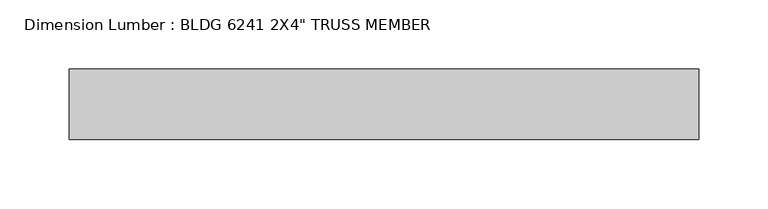
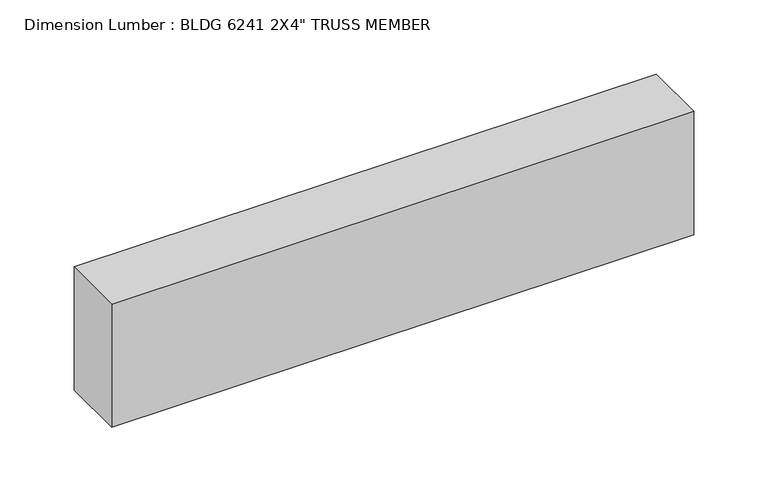
"""IFC4 building model written with IfcOpenShell, lengths in millimetres: beam geometry."""

from ifc_helpers import new_model, si_unit, frame, origin, place, context, project, spatial, polyline, outline, extrude, source, transform, mapped, element, save


def beam_efe25585(model_context):
    return source(origin(), model_context, "Body", "SweptSolid", [
        extrude(outline(polyline([(222.3387319, -25.4), (-231.775, -25.4), (-231.775, 25.4), (222.3387319, 25.4), (222.3387319, -25.4)])), frame((0.0, 0.0, -50.8), z_axis=(0.0, 0.0, 1.0), x_axis=(1.0, 0.0, 0.0)), (0.0, 0.0, 1.0), 101.6),
    ])


if __name__ == "__main__":
    model = new_model("IFC4")
    model_context = context("Model", 3, world=origin())
    ifc_project = project(units=[si_unit("LENGTHUNIT", "METRE", prefix="MILLI")], contexts=[model_context])
    site = spatial("IfcSite", under=ifc_project)
    building = spatial("IfcBuilding", under=site)
    placement = place(None, origin())
    beam_shape = beam_efe25585(model_context)
    element("IfcBeam", 1, ObjectType="Dimension Lumber : BLDG 6241 2X4\" TRUSS MEMBER", at=placement, inside=building, context=model_context, shape_type="MappedRepresentation", body=[
        mapped(beam_shape, transform((0.0, 0.0, 0.0), x_axis=(1.0, 0.0, 0.0), y_axis=(0.0, 1.0, 0.0), z_axis=(0.0, 0.0, 1.0))),
    ])
    save(model, "model.ifc")

# Revit data of these elements
# Type "Dimension Lumber : BLDG 6241 2X4\" TRUSS MEMBER"
#   Assembly Code = "B10"
#   A = 0.273472 SF
#   Length [instance default] = 5' - 0"
#   b = 0' - 2"
#   d = 0' - 4"
#   Structural Material [instance default] = Softwood, Lumber
# Element 1 (IfcBeam, "Dimension Lumber : BLDG 6241 2X4\" TRUSS MEMBER")
#   Materials on its faces: "Softwood, Lumber"
# Materials
#   "Softwood, Lumber": class "Wood", colour RGB 223 192 134, transparency 0, Description = "Pinus Echinata", Cost = 0
